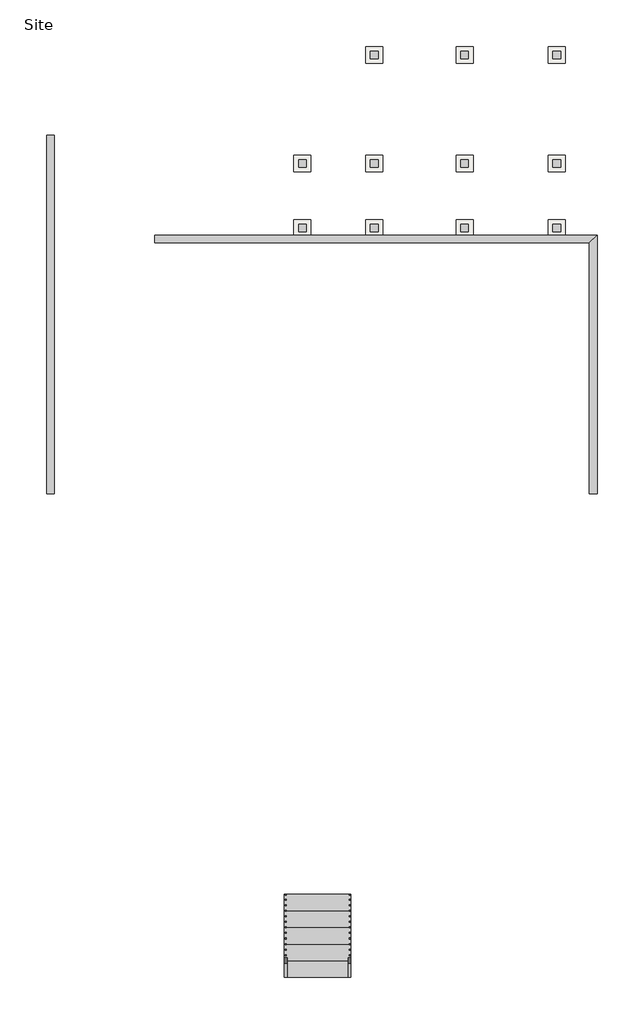
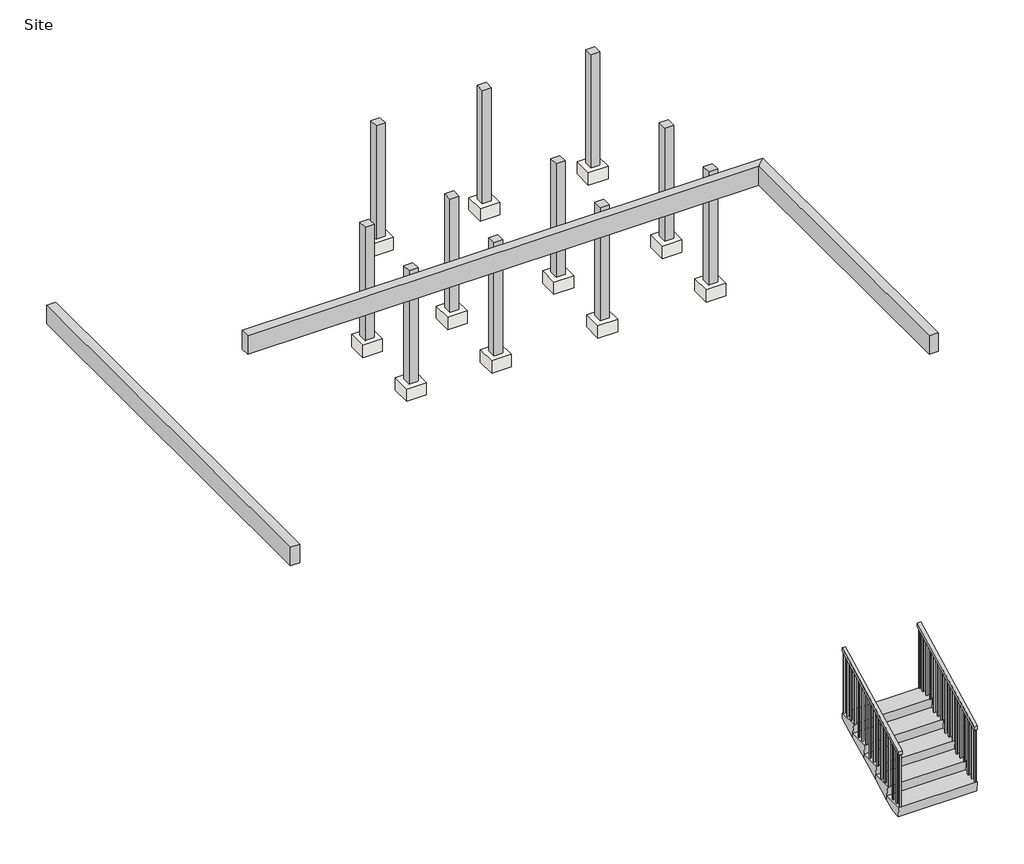
# One storey: 11 columns, 11 slabs, 3 proxies, 2 railings, 1 stair flight.
"""IFC4 building model written with IfcOpenShell, lengths in millimetres."""

import ifcopenshell
import ifcopenshell.guid

model = None  # the IFC model being written
_history = None  # IfcOwnerHistory: only IFC2X3 demands one
_inside = {}  # id of a spatial element -> (the spatial element, [elements in it])
_under = {}  # id of a project, library or spatial element -> (it, [spatial elements below it])
_declared = {}  # id of a project -> (the project, [libraries it declares])
_typed = {}  # id of a type object -> (the type object, [elements of that type])
_made_of = {}  # id of a material, layer set ... -> (it, [elements and type objects made of it])


def new_model(schema):
    """Start an empty IFC model of exactly this schema.

    Asked for "IFC4X3", IfcOpenShell would pick the latest addendum, in which some entities
    have other attributes; the version numbers below select the first issue.
    IFC2X3 requires an IfcOwnerHistory on every rooted entity: one is made here for all.
    """
    global model, _history
    if schema == "IFC4X3":
        model = ifcopenshell.file(schema_version=(4, 3, 0, 0))
    else:
        model = ifcopenshell.file(schema=schema)
    _inside.clear()
    _under.clear()
    _declared.clear()
    _typed.clear()
    _made_of.clear()
    _history = None
    if model.schema == "IFC2X3":
        org = make("IfcOrganization", Name="unknown")
        user = make(
            "IfcPersonAndOrganization",
            ThePerson=make("IfcPerson", FamilyName="unknown"),
            TheOrganization=org,
        )
        app = make(
            "IfcApplication",
            ApplicationDeveloper=org,
            Version="unknown",
            ApplicationFullName="unknown",
            ApplicationIdentifier="unknown",
        )
        _history = make(
            "IfcOwnerHistory",
            OwningUser=user,
            OwningApplication=app,
            ChangeAction="ADDED",
            CreationDate=0,
        )
    return model


def make(cls, **values):
    """One entity of the class cls with the attributes given. An attribute that is None is left unset."""
    return model.create_entity(
        cls, **{name: value for name, value in values.items() if value is not None}
    )


def rooted(cls, **values):
    """An entity with a GlobalId (a new one), such as an element, a storey or a relation."""
    return make(cls, GlobalId=ifcopenshell.guid.new(), OwnerHistory=_history, **values)


def si_unit(unit_type, name, prefix=None):
    """IfcSIUnit, for example si_unit("LENGTHUNIT", "METRE", prefix="MILLI")."""
    return make("IfcSIUnit", UnitType=unit_type, Prefix=prefix, Name=name)


def assignment(units):
    """IfcUnitAssignment: the units of a project."""
    return None if units is None else make("IfcUnitAssignment", Units=units)


def point(xyz):
    """IfcCartesianPoint."""
    return None if xyz is None else make("IfcCartesianPoint", Coordinates=xyz)


def direction(xyz):
    """IfcDirection."""
    return None if xyz is None else make("IfcDirection", DirectionRatios=xyz)


def frame(location, z_axis=None, x_axis=None):
    """IfcAxis2Placement3D, a coordinate frame: its origin and axes. An axis left out is left unset."""
    return make(
        "IfcAxis2Placement3D",
        Location=point(location),
        Axis=direction(z_axis),
        RefDirection=direction(x_axis),
    )


def origin():
    """The frame at (0, 0, 0) with its axes left unset."""
    return frame((0.0, 0.0, 0.0))


def place(relative_to, where):
    """IfcLocalPlacement: puts the frame where relative to a parent placement (None: the world)."""
    return make(
        "IfcLocalPlacement", PlacementRelTo=relative_to, RelativePlacement=where
    )


def context(
    kind, dimensions, precision=None, world=None, true_north=None, identifier=None
):
    """IfcGeometricRepresentationContext, for example the 3D "Model" context."""
    return make(
        "IfcGeometricRepresentationContext",
        ContextIdentifier=identifier,
        ContextType=kind,
        CoordinateSpaceDimension=dimensions,
        Precision=precision,
        WorldCoordinateSystem=world,
        TrueNorth=true_north,
    )


def project(units=None, contexts=None):
    """IfcProject with its units and contexts."""
    return rooted(
        "IfcProject",
        Name="project",
        RepresentationContexts=contexts,
        UnitsInContext=assignment(units),
    )


def spatial(cls, under=None, at=None, **own):
    """A site, building, storey or space (cls), placed at a placement, below another one or the project."""
    s = rooted(cls, ObjectPlacement=at, **own)
    if under is not None:
        _under.setdefault(under.id(), (under, []))[1].append(s)
    return s


def polyline(points):
    """IfcPolyline through the points."""
    return make("IfcPolyline", Points=[point(p) for p in points])


def outline(outer, holes=None, kind="AREA"):
    """IfcArbitraryClosedProfileDef: a profile drawn as a closed curve; with holes, ...WithVoids."""
    if holes is None:
        return make("IfcArbitraryClosedProfileDef", ProfileType=kind, OuterCurve=outer)
    return make(
        "IfcArbitraryProfileDefWithVoids",
        ProfileType=kind,
        OuterCurve=outer,
        InnerCurves=holes,
    )


def extrude(swept, where, along, depth):
    """IfcExtrudedAreaSolid: the profile swept, set in the frame where, extruded along a direction by depth."""
    return make(
        "IfcExtrudedAreaSolid",
        SweptArea=swept,
        Position=where,
        ExtrudedDirection=direction(along),
        Depth=depth,
    )


def faces_of(points, faces, orient=None, outer=None):
    """IfcFace entities. A face is a list of loops; a loop is a list of indices into points, from 0.

    orient and outer hold one flag for each loop. By default every Orientation is true, the
    first loop of a face is its IfcFaceOuterBound and the others are IfcFaceBound.
    """
    made = []
    for i, loops in enumerate(faces):
        bounds = []
        for j, loop in enumerate(loops):
            is_outer = j == 0 if outer is None else outer[i][j]
            bounds.append(
                make(
                    "IfcFaceOuterBound" if is_outer else "IfcFaceBound",
                    Bound=make("IfcPolyLoop", Polygon=[points[k] for k in loop]),
                    Orientation=True if orient is None else orient[i][j],
                )
            )
        made.append(make("IfcFace", Bounds=bounds))
    return made


def faceted_brep(points, faces, orient=None, outer=None, voids=None):
    """IfcFacetedBrep: a solid bounded by flat faces; with voids (closed shells), ...WithVoids."""
    shared = [point(p) for p in points]
    hull = make("IfcClosedShell", CfsFaces=faces_of(shared, faces, orient, outer))
    if voids is None:
        return make("IfcFacetedBrep", Outer=hull)
    return make(
        "IfcFacetedBrepWithVoids",
        Outer=hull,
        Voids=[
            make(cls, CfsFaces=faces_of(shared, fs, o, b)) for cls, fs, o, b in voids
        ],
    )


def shape(context_of_items, identifier, shape_type, items):
    """IfcShapeRepresentation: the items that make up one representation, for example the "Body"."""
    return make(
        "IfcShapeRepresentation",
        ContextOfItems=context_of_items,
        RepresentationIdentifier=identifier,
        RepresentationType=shape_type,
        Items=items,
    )


def source(mapping_origin, context_of_items, identifier, shape_type, items):
    """IfcRepresentationMap: a shape defined once, which mapped items show again and again."""
    return make(
        "IfcRepresentationMap",
        MappingOrigin=mapping_origin,
        MappedRepresentation=shape(context_of_items, identifier, shape_type, items),
    )


def transform(
    local_origin,
    x_axis=None,
    y_axis=None,
    z_axis=None,
    scale=None,
    scale2=None,
    scale3=None,
    uniform=True,
):
    """IfcCartesianTransformationOperator3D, or its non-uniform kind. x_axis, y_axis, z_axis: its Axis1, 2, 3."""
    if uniform:
        return make(
            "IfcCartesianTransformationOperator3D",
            Axis1=direction(x_axis),
            Axis2=direction(y_axis),
            LocalOrigin=point(local_origin),
            Scale=scale,
            Axis3=direction(z_axis),
        )
    return make(
        "IfcCartesianTransformationOperator3DnonUniform",
        Axis1=direction(x_axis),
        Axis2=direction(y_axis),
        LocalOrigin=point(local_origin),
        Scale=scale,
        Axis3=direction(z_axis),
        Scale2=scale2,
        Scale3=scale3,
    )


def mapped(mapping_source, mapping_target):
    """IfcMappedItem: shows the shape of a source again, moved by a transform."""
    return make(
        "IfcMappedItem", MappingSource=mapping_source, MappingTarget=mapping_target
    )


def made_of(thing, what):
    """Note that an element or type object is made of a material, layer set ...; save() writes the relation."""
    if what is not None:
        _made_of.setdefault(what.id(), (what, []))[1].append(thing)
    return thing


def element(
    cls,
    number,
    at=None,
    inside=None,
    cuts=None,
    type_object=None,
    material=None,
    context=None,
    identifier="Body",
    shape_type=None,
    held_by="IfcProductDefinitionShape",
    body=None,
    shapes=None,
    **own,
):
    """One element of the class cls, such as IfcWall. Its Tag is "e" and its number.

    at: its placement. inside: the storey or other place that contains it. cuts: it is an
    opening in that element (IfcRelVoidsElement). A single representation is given by context,
    identifier, shape_type and body (its items); several are given by shapes. held_by: the class
    of the entity that holds the representations. save() writes the other relations.
    """
    e = rooted(cls, Tag="e%d" % number, ObjectPlacement=at, **own)
    if body is not None:
        shapes = [shape(context, identifier, shape_type, body)]
    if shapes is not None:
        e.Representation = make(held_by, Representations=shapes)
    if inside is not None:
        _inside.setdefault(inside.id(), (inside, []))[1].append(e)
    if cuts is not None:
        rooted(
            "IfcRelVoidsElement", RelatingBuildingElement=cuts, RelatedOpeningElement=e
        )
    if type_object is not None:
        _typed.setdefault(type_object.id(), (type_object, []))[1].append(e)
    return made_of(e, material)


def aggregate(whole, parts):
    """IfcRelAggregates: a whole, such as a stair, and the parts it consists of."""
    return rooted("IfcRelAggregates", RelatingObject=whole, RelatedObjects=parts)


def save(model, path):
    """Write the relations noted so far, then the file.

    IfcRelAggregates (storeys below a building ...), IfcRelContainedInSpatialStructure (elements
    in a storey), IfcRelDefinesByType, IfcRelAssociatesMaterial and IfcRelDeclares: one each for
    every whole, place, type object, material and project.
    """
    for whole, parts in _under.values():
        aggregate(whole, parts)
    for where, things in _inside.values():
        rooted(
            "IfcRelContainedInSpatialStructure",
            RelatedElements=things,
            RelatingStructure=where,
        )
    for kind, things in _typed.values():
        rooted("IfcRelDefinesByType", RelatedObjects=things, RelatingType=kind)
    for what, things in _made_of.values():
        rooted("IfcRelAssociatesMaterial", RelatedObjects=things, RelatingMaterial=what)
    for by, libraries in _declared.values():
        rooted("IfcRelDeclares", RelatingContext=by, RelatedDefinitions=libraries)
    model.write(path)


def slab_3d21b0b5(model_context):
    return source(origin(), model_context, "Body", "SweptSolid", [
        extrude(outline(polyline([(152.4, 152.4), (152.4, -152.4), (-152.4, -152.4), (-152.4, 152.4), (152.4, 152.4)])), frame((0.0, 0.0, -203.2), z_axis=(0.0, 0.0, 1.0), x_axis=(1.0, 0.0, 0.0)), (0.0, 0.0, 1.0), 203.2),
    ])


model = new_model("IFC4")

# Units and contexts
model_context = context("Model", 3, world=origin())
ifc_project = project(units=[si_unit("LENGTHUNIT", "METRE", prefix="MILLI")], contexts=[model_context])

# Site, building, storey
site = spatial("IfcSite", under=ifc_project)
building = spatial("IfcBuilding", under=site)
storey = spatial("IfcBuildingStorey", under=building, Name="Site", Elevation=-939.8)

# Proxies
placement = place(None, origin())
element("IfcBuildingElementProxy", 1, Name="Reveals", at=placement, inside=storey, context=model_context, shape_type="SweptSolid", body=[
    extrude(outline(polyline([(-5846.3053068, 3152.0888758), (-5989.1803068, 3152.0888758), (-5989.1803068, 9705.2888758), (-5846.3053068, 9705.2888758), (-5846.3053068, 3152.0888758)])), frame((0.0, 0.0, -654.05), z_axis=(0.0, 0.0, 1.0), x_axis=(1.0, 0.0, 0.0)), (0.0, 0.0, 1.0), 304.8),
])
element("IfcBuildingElementProxy", 2, Name="Reveals", at=placement, inside=storey, context=model_context, shape_type="SweptSolid", body=[
    extrude(outline(polyline([(3926.3446932, 7733.6138758), (4069.2196932, 7876.4888758), (4069.2196932, 3152.0888758), (3926.3446932, 3152.0888758), (3926.3446932, 7733.6138758)])), frame((0.0, 0.0, -654.05), z_axis=(0.0, 0.0, 1.0), x_axis=(1.0, 0.0, 0.0)), (0.0, 0.0, 1.0), 304.8),
])
element("IfcBuildingElementProxy", 3, Name="Reveals", at=placement, inside=storey, context=model_context, shape_type="SweptSolid", body=[
    extrude(outline(polyline([(-4007.9803068, 7733.6138758), (-4007.9803068, 7876.4888758), (4069.2196932, 7876.4888758), (3926.3446932, 7733.6138758), (-4007.9803068, 7733.6138758)])), frame((0.0, 0.0, -654.05), z_axis=(0.0, 0.0, 1.0), x_axis=(1.0, 0.0, 0.0)), (0.0, 0.0, 1.0), 304.8),
])

# Columns
element("IfcColumn", 4, ObjectType="Wood Timber Column : 6 x 6", at=placement, inside=storey, context=model_context, shape_type="SweptSolid", body=[
    extrude(outline(polyline([(-1245.7643654, 9115.1101485), (-1385.4643654, 9115.1101485), (-1385.4643654, 9254.8101485), (-1245.7643654, 9254.8101485), (-1245.7643654, 9115.1101485)])), frame((0.0, 0.0, -2184.4), z_axis=(0.0, 0.0, 1.0), x_axis=(1.0, 0.0, 0.0)), (0.0, 0.0, 1.0), 1860.55),
])
element("IfcColumn", 5, ObjectType="Wood Timber Column : 6 x 6", at=placement, inside=storey, context=model_context, shape_type="SweptSolid", body=[
    extrude(outline(polyline([(69.5237363, 9115.1101485), (-70.1762637, 9115.1101485), (-70.1762637, 9254.8101485), (69.5237363, 9254.8101485), (69.5237363, 9115.1101485)])), frame((0.0, 0.0, -2184.4), z_axis=(0.0, 0.0, 1.0), x_axis=(1.0, 0.0, 0.0)), (0.0, 0.0, 1.0), 1860.55),
])
element("IfcColumn", 6, ObjectType="Wood Timber Column : 6 x 6", at=placement, inside=storey, context=model_context, shape_type="SweptSolid", body=[
    extrude(outline(polyline([(69.5237363, 11099.8562662), (-70.1762637, 11099.8562662), (-70.1762637, 11239.5562662), (69.5237363, 11239.5562662), (69.5237363, 11099.8562662)])), frame((0.0, 0.0, -2184.4), z_axis=(0.0, 0.0, 1.0), x_axis=(1.0, 0.0, 0.0)), (0.0, 0.0, 1.0), 1860.55),
])
element("IfcColumn", 7, ObjectType="Wood Timber Column : 6 x 6", at=placement, inside=storey, context=model_context, shape_type="SweptSolid", body=[
    extrude(outline(polyline([(1720.2890638, 11099.8562662), (1580.5890638, 11099.8562662), (1580.5890638, 11239.5562662), (1720.2890638, 11239.5562662), (1720.2890638, 11099.8562662)])), frame((0.0, 0.0, -2184.4), z_axis=(0.0, 0.0, 1.0), x_axis=(1.0, 0.0, 0.0)), (0.0, 0.0, 1.0), 1860.55),
])
element("IfcColumn", 8, ObjectType="Wood Timber Column : 6 x 6", at=placement, inside=storey, context=model_context, shape_type="SweptSolid", body=[
    extrude(outline(polyline([(3402.4696932, 11099.8562662), (3262.7696932, 11099.8562662), (3262.7696932, 11239.5562662), (3402.4696932, 11239.5562662), (3402.4696932, 11099.8562662)])), frame((0.0, 0.0, -2184.4), z_axis=(0.0, 0.0, 1.0), x_axis=(1.0, 0.0, 0.0)), (0.0, 0.0, 1.0), 1860.55),
])
element("IfcColumn", 9, ObjectType="Wood Timber Column : 6 x 6", at=placement, inside=storey, context=model_context, shape_type="SweptSolid", body=[
    extrude(outline(polyline([(3402.4696932, 9115.1101485), (3262.7696932, 9115.1101485), (3262.7696932, 9254.8101485), (3402.4696932, 9254.8101485), (3402.4696932, 9115.1101485)])), frame((0.0, 0.0, -2184.4), z_axis=(0.0, 0.0, 1.0), x_axis=(1.0, 0.0, 0.0)), (0.0, 0.0, 1.0), 1860.55),
])
element("IfcColumn", 10, ObjectType="Wood Timber Column : 6 x 6", at=placement, inside=storey, context=model_context, shape_type="SweptSolid", body=[
    extrude(outline(polyline([(3402.4696932, 7933.6388758), (3262.7696932, 7933.6388758), (3262.7696932, 8073.3388758), (3402.4696932, 8073.3388758), (3402.4696932, 7933.6388758)])), frame((0.0, 0.0, -2184.4), z_axis=(0.0, 0.0, 1.0), x_axis=(1.0, 0.0, 0.0)), (0.0, 0.0, 1.0), 1860.55),
])
element("IfcColumn", 11, ObjectType="Wood Timber Column : 6 x 6", at=placement, inside=storey, context=model_context, shape_type="SweptSolid", body=[
    extrude(outline(polyline([(-1245.7643654, 7933.6388758), (-1385.4643654, 7933.6388758), (-1385.4643654, 8073.3388758), (-1245.7643654, 8073.3388758), (-1245.7643654, 7933.6388758)])), frame((0.0, 0.0, -2184.4), z_axis=(0.0, 0.0, 1.0), x_axis=(1.0, 0.0, 0.0)), (0.0, 0.0, 1.0), 1860.55),
])
element("IfcColumn", 12, ObjectType="Wood Timber Column : 6 x 6", at=placement, inside=storey, context=model_context, shape_type="SweptSolid", body=[
    extrude(outline(polyline([(69.5237363, 7933.6388758), (-70.1762637, 7933.6388758), (-70.1762637, 8073.3388758), (69.5237363, 8073.3388758), (69.5237363, 7933.6388758)])), frame((0.0, 0.0, -2184.4), z_axis=(0.0, 0.0, 1.0), x_axis=(1.0, 0.0, 0.0)), (0.0, 0.0, 1.0), 1860.55),
])
element("IfcColumn", 13, ObjectType="Wood Timber Column : 6 x 6", at=placement, inside=storey, context=model_context, shape_type="SweptSolid", body=[
    extrude(outline(polyline([(1720.2890638, 9115.1101485), (1580.5890638, 9115.1101485), (1580.5890638, 9254.8101485), (1720.2890638, 9254.8101485), (1720.2890638, 9115.1101485)])), frame((0.0, 0.0, -2184.4), z_axis=(0.0, 0.0, 1.0), x_axis=(1.0, 0.0, 0.0)), (0.0, 0.0, 1.0), 1860.55),
])
element("IfcColumn", 14, ObjectType="Wood Timber Column : 6 x 6", at=placement, inside=storey, context=model_context, shape_type="SweptSolid", body=[
    extrude(outline(polyline([(1720.2890638, 7933.6388758), (1580.5890638, 7933.6388758), (1580.5890638, 8073.3388758), (1720.2890638, 8073.3388758), (1720.2890638, 7933.6388758)])), frame((0.0, 0.0, -2184.4), z_axis=(0.0, 0.0, 1.0), x_axis=(1.0, 0.0, 0.0)), (0.0, 0.0, 1.0), 1860.55),
])

# Railings
element("IfcRailing", 15, ObjectType="Handrail - Rectangular", at=placement, inside=storey, context=model_context, shape_type="SweptSolid", body=[
    extrude(outline(polyline([(-5687.1111242, 74.1181862), (-5687.1111242, 131.2333333), (-4163.1111242, 914.4), (-4163.1111242, 857.2848529), (-5687.1111242, 74.1181862)])), frame((-477.3803068, 0.0, 0.0), z_axis=(1.0, 0.0, 0.0), x_axis=(0.0, 1.0, 0.0)), (0.0, 0.0, 1.0), 50.8),
    extrude(outline(polyline([(-4274.2361242, 800.1789501), (-4255.1861242, 809.9685334), (-4255.1861242, -156.6333333), (-4274.2361242, -156.6333333), (-4274.2361242, 800.1789501)])), frame((-461.5053068, 0.0, 0.0), z_axis=(1.0, 0.0, 0.0), x_axis=(0.0, 1.0, 0.0)), (0.0, 0.0, 1.0), 19.05),
    extrude(outline(polyline([(-4375.8361242, 747.967839), (-4356.7861242, 757.7574223), (-4356.7861242, -156.6333333), (-4375.8361242, -156.6333333), (-4375.8361242, 747.967839)])), frame((-461.5053068, 0.0, 0.0), z_axis=(1.0, 0.0, 0.0), x_axis=(0.0, 1.0, 0.0)), (0.0, 0.0, 1.0), 19.05),
    extrude(outline(polyline([(-4477.4361242, 695.7567279), (-4458.3861242, 705.5463112), (-4458.3861242, -156.6333333), (-4477.4361242, -156.6333333), (-4477.4361242, 695.7567279)])), frame((-461.5053068, 0.0, 0.0), z_axis=(1.0, 0.0, 0.0), x_axis=(0.0, 1.0, 0.0)), (0.0, 0.0, 1.0), 19.05),
    extrude(outline(polyline([(-4579.0361242, 643.5456168), (-4559.9861242, 653.3352001), (-4559.9861242, -313.2666667), (-4579.0361242, -313.2666667), (-4579.0361242, 643.5456168)])), frame((-461.5053068, 0.0, 0.0), z_axis=(1.0, 0.0, 0.0), x_axis=(0.0, 1.0, 0.0)), (0.0, 0.0, 1.0), 19.05),
    extrude(outline(polyline([(-4680.6361242, 591.3345057), (-4661.5861242, 601.124089), (-4661.5861242, -313.2666667), (-4680.6361242, -313.2666667), (-4680.6361242, 591.3345057)])), frame((-461.5053068, 0.0, 0.0), z_axis=(1.0, 0.0, 0.0), x_axis=(0.0, 1.0, 0.0)), (0.0, 0.0, 1.0), 19.05),
    extrude(outline(polyline([(-4782.2361242, 539.1233945), (-4763.1861242, 548.9129779), (-4763.1861242, -313.2666667), (-4782.2361242, -313.2666667), (-4782.2361242, 539.1233945)])), frame((-461.5053068, 0.0, 0.0), z_axis=(1.0, 0.0, 0.0), x_axis=(0.0, 1.0, 0.0)), (0.0, 0.0, 1.0), 19.05),
    extrude(outline(polyline([(-4883.8361242, 486.9122834), (-4864.7861242, 496.7018668), (-4864.7861242, -469.9), (-4883.8361242, -469.9), (-4883.8361242, 486.9122834)])), frame((-461.5053068, 0.0, 0.0), z_axis=(1.0, 0.0, 0.0), x_axis=(0.0, 1.0, 0.0)), (0.0, 0.0, 1.0), 19.05),
    extrude(outline(polyline([(-4985.4361242, 434.7011723), (-4966.3861242, 444.4907557), (-4966.3861242, -469.9), (-4985.4361242, -469.9), (-4985.4361242, 434.7011723)])), frame((-461.5053068, 0.0, 0.0), z_axis=(1.0, 0.0, 0.0), x_axis=(0.0, 1.0, 0.0)), (0.0, 0.0, 1.0), 19.05),
    extrude(outline(polyline([(-5087.0361242, 382.4900612), (-5067.9861242, 392.2796445), (-5067.9861242, -469.9), (-5087.0361242, -469.9), (-5087.0361242, 382.4900612)])), frame((-461.5053068, 0.0, 0.0), z_axis=(1.0, 0.0, 0.0), x_axis=(0.0, 1.0, 0.0)), (0.0, 0.0, 1.0), 19.05),
    extrude(outline(polyline([(-5188.6361242, 330.2789501), (-5169.5861242, 340.0685334), (-5169.5861242, -626.5333333), (-5188.6361242, -626.5333333), (-5188.6361242, 330.2789501)])), frame((-461.5053068, 0.0, 0.0), z_axis=(1.0, 0.0, 0.0), x_axis=(0.0, 1.0, 0.0)), (0.0, 0.0, 1.0), 19.05),
    extrude(outline(polyline([(-5290.2361242, 278.067839), (-5271.1861242, 287.8574223), (-5271.1861242, -626.5333333), (-5290.2361242, -626.5333333), (-5290.2361242, 278.067839)])), frame((-461.5053068, 0.0, 0.0), z_axis=(1.0, 0.0, 0.0), x_axis=(0.0, 1.0, 0.0)), (0.0, 0.0, 1.0), 19.05),
    extrude(outline(polyline([(-5391.8361242, 225.8567279), (-5372.7861242, 235.6463112), (-5372.7861242, -626.5333333), (-5391.8361242, -626.5333333), (-5391.8361242, 225.8567279)])), frame((-461.5053068, 0.0, 0.0), z_axis=(1.0, 0.0, 0.0), x_axis=(0.0, 1.0, 0.0)), (0.0, 0.0, 1.0), 19.05),
    extrude(outline(polyline([(-5493.4361242, 173.6456168), (-5474.3861242, 183.4352001), (-5474.3861242, -783.1666667), (-5493.4361242, -783.1666667), (-5493.4361242, 173.6456168)])), frame((-461.5053068, 0.0, 0.0), z_axis=(1.0, 0.0, 0.0), x_axis=(0.0, 1.0, 0.0)), (0.0, 0.0, 1.0), 19.05),
    extrude(outline(polyline([(-5595.0361242, 121.4345057), (-5575.9861242, 131.224089), (-5575.9861242, -783.1666667), (-5595.0361242, -783.1666667), (-5595.0361242, 121.4345057)])), frame((-461.5053068, 0.0, 0.0), z_axis=(1.0, 0.0, 0.0), x_axis=(0.0, 1.0, 0.0)), (0.0, 0.0, 1.0), 19.05),
    extrude(outline(polyline([(-4182.1611242, 847.4952695), (-4163.1111242, 857.2848529), (-4163.1111242, -156.6333333), (-4182.1611242, -156.6333333), (-4182.1611242, 847.4952695)])), frame((-461.5053068, 0.0, 0.0), z_axis=(1.0, 0.0, 0.0), x_axis=(0.0, 1.0, 0.0)), (0.0, 0.0, 1.0), 19.05),
    extrude(outline(polyline([(-5687.1111242, 74.1181862), (-5668.0611242, 83.9077695), (-5668.0611242, -783.1666667), (-5687.1111242, -783.1666667), (-5687.1111242, 74.1181862)])), frame((-461.5053068, 0.0, 0.0), z_axis=(1.0, 0.0, 0.0), x_axis=(0.0, 1.0, 0.0)), (0.0, 0.0, 1.0), 19.05),
])
element("IfcRailing", 16, ObjectType="Handrail - Rectangular", at=placement, inside=storey, context=model_context, shape_type="SweptSolid", body=[
    extrude(outline(polyline([(-5687.1111242, 74.1181862), (-5687.1111242, 131.2333333), (-4163.1111242, 914.4), (-4163.1111242, 857.2848529), (-5687.1111242, 74.1181862)])), frame((-1645.7803068, 0.0, 0.0), z_axis=(1.0, 0.0, 0.0), x_axis=(0.0, 1.0, 0.0)), (0.0, 0.0, 1.0), 50.8),
    extrude(outline(polyline([(-4255.1861242, 809.9685334), (-4255.1861242, -156.6333333), (-4274.2361242, -156.6333333), (-4274.2361242, 800.1789501), (-4255.1861242, 809.9685334)])), frame((-1629.9053068, 0.0, 0.0), z_axis=(1.0, 0.0, 0.0), x_axis=(0.0, 1.0, 0.0)), (0.0, 0.0, 1.0), 19.05),
    extrude(outline(polyline([(-4356.7861242, 757.7574223), (-4356.7861242, -156.6333333), (-4375.8361242, -156.6333333), (-4375.8361242, 747.967839), (-4356.7861242, 757.7574223)])), frame((-1629.9053068, 0.0, 0.0), z_axis=(1.0, 0.0, 0.0), x_axis=(0.0, 1.0, 0.0)), (0.0, 0.0, 1.0), 19.05),
    extrude(outline(polyline([(-4458.3861242, 705.5463112), (-4458.3861242, -156.6333333), (-4477.4361242, -156.6333333), (-4477.4361242, 695.7567279), (-4458.3861242, 705.5463112)])), frame((-1629.9053068, 0.0, 0.0), z_axis=(1.0, 0.0, 0.0), x_axis=(0.0, 1.0, 0.0)), (0.0, 0.0, 1.0), 19.05),
    extrude(outline(polyline([(-4559.9861242, 653.3352001), (-4559.9861242, -313.2666667), (-4579.0361242, -313.2666667), (-4579.0361242, 643.5456168), (-4559.9861242, 653.3352001)])), frame((-1629.9053068, 0.0, 0.0), z_axis=(1.0, 0.0, 0.0), x_axis=(0.0, 1.0, 0.0)), (0.0, 0.0, 1.0), 19.05),
    extrude(outline(polyline([(-4661.5861242, 601.124089), (-4661.5861242, -313.2666667), (-4680.6361242, -313.2666667), (-4680.6361242, 591.3345057), (-4661.5861242, 601.124089)])), frame((-1629.9053068, 0.0, 0.0), z_axis=(1.0, 0.0, 0.0), x_axis=(0.0, 1.0, 0.0)), (0.0, 0.0, 1.0), 19.05),
    extrude(outline(polyline([(-4763.1861242, 548.9129779), (-4763.1861242, -313.2666667), (-4782.2361242, -313.2666667), (-4782.2361242, 539.1233945), (-4763.1861242, 548.9129779)])), frame((-1629.9053068, 0.0, 0.0), z_axis=(1.0, 0.0, 0.0), x_axis=(0.0, 1.0, 0.0)), (0.0, 0.0, 1.0), 19.05),
    extrude(outline(polyline([(-4864.7861242, 496.7018668), (-4864.7861242, -469.9), (-4883.8361242, -469.9), (-4883.8361242, 486.9122834), (-4864.7861242, 496.7018668)])), frame((-1629.9053068, 0.0, 0.0), z_axis=(1.0, 0.0, 0.0), x_axis=(0.0, 1.0, 0.0)), (0.0, 0.0, 1.0), 19.05),
    extrude(outline(polyline([(-4966.3861242, 444.4907557), (-4966.3861242, -469.9), (-4985.4361242, -469.9), (-4985.4361242, 434.7011723), (-4966.3861242, 444.4907557)])), frame((-1629.9053068, 0.0, 0.0), z_axis=(1.0, 0.0, 0.0), x_axis=(0.0, 1.0, 0.0)), (0.0, 0.0, 1.0), 19.05),
    extrude(outline(polyline([(-5067.9861242, 392.2796445), (-5067.9861242, -469.9), (-5087.0361242, -469.9), (-5087.0361242, 382.4900612), (-5067.9861242, 392.2796445)])), frame((-1629.9053068, 0.0, 0.0), z_axis=(1.0, 0.0, 0.0), x_axis=(0.0, 1.0, 0.0)), (0.0, 0.0, 1.0), 19.05),
    extrude(outline(polyline([(-5169.5861242, 340.0685334), (-5169.5861242, -626.5333333), (-5188.6361242, -626.5333333), (-5188.6361242, 330.2789501), (-5169.5861242, 340.0685334)])), frame((-1629.9053068, 0.0, 0.0), z_axis=(1.0, 0.0, 0.0), x_axis=(0.0, 1.0, 0.0)), (0.0, 0.0, 1.0), 19.05),
    extrude(outline(polyline([(-5271.1861242, 287.8574223), (-5271.1861242, -626.5333333), (-5290.2361242, -626.5333333), (-5290.2361242, 278.067839), (-5271.1861242, 287.8574223)])), frame((-1629.9053068, 0.0, 0.0), z_axis=(1.0, 0.0, 0.0), x_axis=(0.0, 1.0, 0.0)), (0.0, 0.0, 1.0), 19.05),
    extrude(outline(polyline([(-5372.7861242, 235.6463112), (-5372.7861242, -626.5333333), (-5391.8361242, -626.5333333), (-5391.8361242, 225.8567279), (-5372.7861242, 235.6463112)])), frame((-1629.9053068, 0.0, 0.0), z_axis=(1.0, 0.0, 0.0), x_axis=(0.0, 1.0, 0.0)), (0.0, 0.0, 1.0), 19.05),
    extrude(outline(polyline([(-5474.3861242, 183.4352001), (-5474.3861242, -783.1666667), (-5493.4361242, -783.1666667), (-5493.4361242, 173.6456168), (-5474.3861242, 183.4352001)])), frame((-1629.9053068, 0.0, 0.0), z_axis=(1.0, 0.0, 0.0), x_axis=(0.0, 1.0, 0.0)), (0.0, 0.0, 1.0), 19.05),
    extrude(outline(polyline([(-5575.9861242, 131.224089), (-5575.9861242, -783.1666667), (-5595.0361242, -783.1666667), (-5595.0361242, 121.4345057), (-5575.9861242, 131.224089)])), frame((-1629.9053068, 0.0, 0.0), z_axis=(1.0, 0.0, 0.0), x_axis=(0.0, 1.0, 0.0)), (0.0, 0.0, 1.0), 19.05),
    extrude(outline(polyline([(-4163.1111242, 857.2848529), (-4163.1111242, -156.6333333), (-4182.1611242, -156.6333333), (-4182.1611242, 847.4952695), (-4163.1111242, 857.2848529)])), frame((-1629.9053068, 0.0, 0.0), z_axis=(1.0, 0.0, 0.0), x_axis=(0.0, 1.0, 0.0)), (0.0, 0.0, 1.0), 19.05),
    extrude(outline(polyline([(-5668.0611242, 83.9077695), (-5668.0611242, -783.1666667), (-5687.1111242, -783.1666667), (-5687.1111242, 74.1181862), (-5668.0611242, 83.9077695)])), frame((-1629.9053068, 0.0, 0.0), z_axis=(1.0, 0.0, 0.0), x_axis=(0.0, 1.0, 0.0)), (0.0, 0.0, 1.0), 19.05),
])

# Slabs
slab_shape = slab_3d21b0b5(model_context)
element("IfcSlab", 17, ObjectType="Footing-Rectangular : 12\" x 12\" x 8\"", at=placement, inside=storey, context=model_context, shape_type="MappedRepresentation", body=[
    mapped(slab_shape, transform((3332.6196932, 9184.9601485, -2184.4), x_axis=(-1.0, 0.0, 0.0), y_axis=(0.0, -1.0, 0.0), z_axis=(0.0, 0.0, 1.0))),
])
element("IfcSlab", 18, ObjectType="Footing-Rectangular : 12\" x 12\" x 8\"", at=placement, inside=storey, context=model_context, shape_type="MappedRepresentation", body=[
    mapped(slab_shape, transform((1650.4390638, 9184.9601485, -2184.4), x_axis=(-1.0, 0.0, 0.0), y_axis=(0.0, -1.0, 0.0), z_axis=(0.0, 0.0, 1.0))),
])
element("IfcSlab", 19, ObjectType="Footing-Rectangular : 12\" x 12\" x 8\"", at=placement, inside=storey, context=model_context, shape_type="MappedRepresentation", body=[
    mapped(slab_shape, transform((-0.3262637, 9184.9601485, -2184.4), x_axis=(-1.0, 0.0, 0.0), y_axis=(0.0, -1.0, 0.0), z_axis=(0.0, 0.0, 1.0))),
])
element("IfcSlab", 20, ObjectType="Footing-Rectangular : 12\" x 12\" x 8\"", at=placement, inside=storey, context=model_context, shape_type="MappedRepresentation", body=[
    mapped(slab_shape, transform((-1315.6143654, 9184.9601485, -2184.4), x_axis=(-1.0, 0.0, 0.0), y_axis=(0.0, -1.0, 0.0), z_axis=(0.0, 0.0, 1.0))),
])
element("IfcSlab", 21, ObjectType="Footing-Rectangular : 12\" x 12\" x 8\"", at=placement, inside=storey, context=model_context, shape_type="MappedRepresentation", body=[
    mapped(slab_shape, transform((-1315.6143654, 8003.4888758, -2184.4), x_axis=(-1.0, 0.0, 0.0), y_axis=(0.0, -1.0, 0.0), z_axis=(0.0, 0.0, 1.0))),
])
element("IfcSlab", 22, ObjectType="Footing-Rectangular : 12\" x 12\" x 8\"", at=placement, inside=storey, context=model_context, shape_type="MappedRepresentation", body=[
    mapped(slab_shape, transform((-0.3262637, 8003.4888758, -2184.4), x_axis=(-1.0, 0.0, 0.0), y_axis=(0.0, -1.0, 0.0), z_axis=(0.0, 0.0, 1.0))),
])
element("IfcSlab", 23, ObjectType="Footing-Rectangular : 12\" x 12\" x 8\"", at=placement, inside=storey, context=model_context, shape_type="MappedRepresentation", body=[
    mapped(slab_shape, transform((1650.4390638, 8003.4888758, -2184.4), x_axis=(-1.0, 0.0, 0.0), y_axis=(0.0, -1.0, 0.0), z_axis=(0.0, 0.0, 1.0))),
])
element("IfcSlab", 24, ObjectType="Footing-Rectangular : 12\" x 12\" x 8\"", at=placement, inside=storey, context=model_context, shape_type="MappedRepresentation", body=[
    mapped(slab_shape, transform((3332.6196932, 8003.4888758, -2184.4), x_axis=(-1.0, 0.0, 0.0), y_axis=(0.0, -1.0, 0.0), z_axis=(0.0, 0.0, 1.0))),
])
element("IfcSlab", 25, ObjectType="Footing-Rectangular : 12\" x 12\" x 8\"", at=placement, inside=storey, context=model_context, shape_type="MappedRepresentation", body=[
    mapped(slab_shape, transform((3332.6196932, 11169.7062662, -2184.4), x_axis=(-1.0, 0.0, 0.0), y_axis=(0.0, -1.0, 0.0), z_axis=(0.0, 0.0, 1.0))),
])
element("IfcSlab", 26, ObjectType="Footing-Rectangular : 12\" x 12\" x 8\"", at=placement, inside=storey, context=model_context, shape_type="MappedRepresentation", body=[
    mapped(slab_shape, transform((1650.4390638, 11169.7062662, -2184.4), x_axis=(-1.0, 0.0, 0.0), y_axis=(0.0, -1.0, 0.0), z_axis=(0.0, 0.0, 1.0))),
])
element("IfcSlab", 27, ObjectType="Footing-Rectangular : 12\" x 12\" x 8\"", at=placement, inside=storey, context=model_context, shape_type="MappedRepresentation", body=[
    mapped(slab_shape, transform((-0.3262637, 11169.7062662, -2184.4), x_axis=(-1.0, 0.0, 0.0), y_axis=(0.0, -1.0, 0.0), z_axis=(0.0, 0.0, 1.0))),
])

# Stair flight
element("IfcStairFlight", 28, ObjectType="3/4\" Nosing", at=placement, inside=storey, context=model_context, shape_type="Brep", body=[
    faceted_brep([(-426.5803068, -5687.1111242, -783.1666667), (-1645.7803068, -5687.1111242, -783.1666667), (-1645.7803068, -5668.0611242, -939.8), (-426.5803068, -5668.0611242, -939.8), (-426.5803068, -5363.2611242, -783.1666667), (-1645.7803068, -5363.2611242, -783.1666667), (-1645.7803068, -5363.2611242, -854.5606006), (-1645.7803068, -5529.1323879, -939.8), (-426.5803068, -5529.1323879, -939.8), (-426.5803068, -5363.2611242, -854.5606006), (-1645.7803068, -5382.3111242, -626.5333333), (-426.5803068, -5382.3111242, -626.5333333), (-426.5803068, -5058.4611242, -626.5333333), (-1645.7803068, -5058.4611242, -626.5333333), (-1645.7803068, -5058.4611242, -697.9272672), (-426.5803068, -5058.4611242, -697.9272672), (-1645.7803068, -5077.5111242, -469.9), (-426.5803068, -5077.5111242, -469.9), (-426.5803068, -4753.6611242, -469.9), (-1645.7803068, -4753.6611242, -469.9), (-1645.7803068, -4753.6611242, -541.2939339), (-426.5803068, -4753.6611242, -541.2939339), (-1645.7803068, -4772.7111242, -313.2666667), (-426.5803068, -4772.7111242, -313.2666667), (-426.5803068, -4448.8611242, -313.2666667), (-1645.7803068, -4448.8611242, -313.2666667), (-1645.7803068, -4448.8611242, -384.6606006), (-426.5803068, -4448.8611242, -384.6606006), (-1645.7803068, -4467.9111242, -156.6333333), (-426.5803068, -4467.9111242, -156.6333333), (-426.5803068, -4163.1111242, -156.6333333), (-1645.7803068, -4163.1111242, -156.6333333), (-1645.7803068, -4163.1111242, -237.8168506), (-426.5803068, -4163.1111242, -237.8168506)], [[[0, 1, 2, 3]], [[1, 0, 4, 5]], [[1, 5, 6, 7, 2]], [[4, 0, 3, 8, 9]], [[10, 11, 12, 13]], [[10, 13, 14, 6, 5]], [[12, 11, 4, 9, 15]], [[5, 4, 11, 10]], [[16, 17, 18, 19]], [[16, 19, 20, 14, 13]], [[18, 17, 12, 15, 21]], [[13, 12, 17, 16]], [[22, 23, 24, 25]], [[22, 25, 26, 20, 19]], [[24, 23, 18, 21, 27]], [[19, 18, 23, 22]], [[28, 29, 30, 31]], [[28, 31, 32, 26, 25]], [[30, 29, 24, 27, 33]], [[31, 30, 33, 32]], [[25, 24, 29, 28]], [[3, 2, 7, 8]], [[8, 7, 6, 14, 20, 26, 32, 33, 27, 21, 15, 9]]]),
])

save(model, "model.ifc")

# Revit data of these elements
# Type "Wood Timber Column : 6 x 6"
#   Assembly Code = "B1010200"
#   Depth = 0' - 5 1/2"
#   Width = 0' - 5 1/2"
#   Material = Wood - Dimensional lumber
# Type "Handrail - Rectangular"
#   Assembly Code = "C2010400"
#   built-in parameter 1008612 = 0.0416667 (stored number, unit not read)
#   built-in parameter 1008611 = 0.0416667 (stored number, unit not read)
#   built-in parameter 1008609 = 0.333333 (stored number, unit not read)
#   built-in parameter 1008604 = 0.166667 (stored number, unit not read)
#   built-in parameter 1008603 = 0.166667 (stored number, unit not read)
#   Railing Height = 3' - 0"
#   built-in parameter 1008630 = 2
#   built-in parameter 1008610 = 2
#   built-in parameter 1008618 = Baluster - Square : 3/4"
# Type "Footing-Rectangular : 12\" x 12\" x 8\""
#   Assembly Code = "A1010100"
#   Width = 1' - 0"
#   Length = 1' - 0"
#   Thickness = 0' - 8"
#   Structural Material [instance default] = Concrete - Cast-in-Place Concrete
# Elements 4, 5, 6, 7, 8, 9, 10, 11, 12, 13, 14 (IfcColumn, "Wood Timber Column : 6 x 6")
#   Phase Created = New Construction
#   Materials on its faces: "Wood - Dimensional lumber"
# Elements 15, 16 (IfcRailing, "Handrail - Rectangular")
#   Phase Created = Existing
# Elements 17, 18, 19, 20, 21, 22, 23, 24, 25, 26, 27 (IfcSlab, "Footing-Rectangular : 12\" x 12\" x 8\"")
#   Elevation at Bottom = none
#   Phase Created = New Construction
#   Materials on its faces: "Concrete - Cast-in-Place Concrete"
# Element 28 (IfcStairFlight, "3/4\" Nosing")
#   Phase Created = Existing
#   Materials on its faces: "Concrete, Cast-in-Place gray"
# Materials
#   "Wood - Dimensional lumber": class "Unassigned", colour RGB 223 192 134, transparency 0
#   "Concrete - Cast-in-Place Concrete": class "Unassigned", colour RGB 192 192 192, transparency 0
#   "Concrete, Cast-in-Place gray": class "Concrete", colour RGB 192 192 192, transparency 0, Description = "Cast-in-place concrete", Cost = 0
